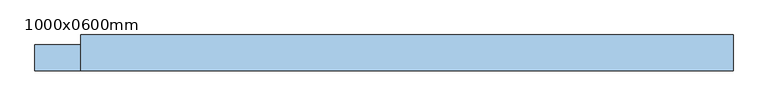
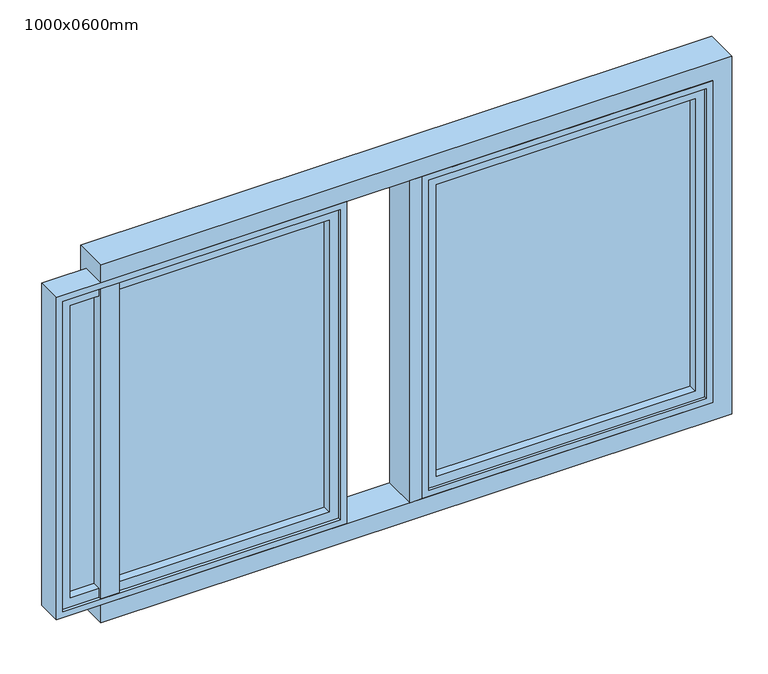
"""IFC4 building model written with IfcOpenShell, lengths in millimetres: window geometry, Janela Maxim-air - 2 Módulos : 1000x0600mm."""

from ifc_helpers import new_model, si_unit, frame, origin, place, context, project, spatial, polyline, outline, extrude, faceted_brep, source, transform, mapped, element, save


def window_1000x0600mm_9fc04acc(model_context):
    return source(origin(), model_context, "Body", "SolidModel", [
        extrude(outline(polyline([(452.0, 51.3), (28.0, 51.3), (28.0, 58.3), (452.0, 58.3), (452.0, 51.3)])), frame((0.0, 0.0, 1048.0), z_axis=(0.0, 0.0, 1.0), x_axis=(1.0, 0.0, 0.0)), (0.0, 0.0, 1.0), 504.0),
        faceted_brep([(35.0, 72.3, 1545.0), (35.0, 58.3, 1545.0), (35.0, 58.3, 1055.0), (35.0, 72.3, 1055.0), (28.0, 58.3, 1552.0), (28.0, 51.3, 1552.0), (28.0, 51.3, 1048.0), (28.0, 58.3, 1048.0), (35.0, 51.3, 1545.0), (35.0, 37.3, 1545.0), (35.0, 37.3, 1055.0), (35.0, 51.3, 1055.0), (15.0, 37.3, 1565.0), (15.0, 72.3, 1565.0), (15.0, 72.3, 1035.0), (15.0, 37.3, 1035.0), (445.0, 58.3, 1055.0), (445.0, 72.3, 1055.0), (452.0, 51.3, 1048.0), (452.0, 58.3, 1048.0), (445.0, 37.3, 1055.0), (445.0, 51.3, 1055.0), (465.0, 72.3, 1035.0), (465.0, 37.3, 1035.0), (445.0, 58.3, 1545.0), (445.0, 72.3, 1545.0), (452.0, 51.3, 1552.0), (452.0, 58.3, 1552.0), (445.0, 37.3, 1545.0), (445.0, 51.3, 1545.0), (465.0, 72.3, 1565.0), (465.0, 37.3, 1565.0)], [[[0, 1, 2, 3]], [[4, 5, 6, 7]], [[8, 9, 10, 11]], [[12, 13, 14, 15]], [[3, 2, 16, 17]], [[7, 6, 18, 19]], [[11, 10, 20, 21]], [[15, 14, 22, 23]], [[17, 16, 24, 25]], [[19, 18, 26, 27]], [[21, 20, 28, 29]], [[23, 22, 30, 31]], [[13, 30, 22, 14], [3, 17, 25, 0]], [[25, 24, 1, 0]], [[7, 19, 27, 4], [1, 24, 16, 2]], [[27, 26, 5, 4]], [[5, 26, 18, 6], [11, 21, 29, 8]], [[29, 28, 9, 8]], [[15, 23, 31, 12], [9, 28, 20, 10]], [[31, 30, 13, 12]]]),
        faceted_brep([(15.0, 72.3, 1565.0), (15.0, 37.3, 1565.0), (15.0, 37.3, 1035.0), (15.0, 72.3, 1035.0), (20.0, 37.3, 1560.0), (20.0, 32.3, 1560.0), (20.0, 32.3, 1040.0), (20.0, 37.3, 1040.0), (10.0, 32.3, 1570.0), (10.0, 72.3, 1570.0), (10.0, 72.3, 1030.0), (10.0, 32.3, 1030.0), (465.0, 37.3, 1035.0), (465.0, 72.3, 1035.0), (460.0, 32.3, 1040.0), (460.0, 37.3, 1040.0), (470.0, 72.3, 1030.0), (470.0, 32.3, 1030.0), (465.0, 37.3, 1565.0), (465.0, 72.3, 1565.0), (460.0, 32.3, 1560.0), (460.0, 37.3, 1560.0), (470.0, 72.3, 1570.0), (470.0, 32.3, 1570.0)], [[[0, 1, 2, 3]], [[4, 5, 6, 7]], [[8, 9, 10, 11]], [[3, 2, 12, 13]], [[7, 6, 14, 15]], [[11, 10, 16, 17]], [[13, 12, 18, 19]], [[15, 14, 20, 21]], [[17, 16, 22, 23]], [[9, 22, 16, 10], [3, 13, 19, 0]], [[19, 18, 1, 0]], [[1, 18, 12, 2], [7, 15, 21, 4]], [[21, 20, 5, 4]], [[11, 17, 23, 8], [5, 20, 14, 6]], [[23, 22, 9, 8]]]),
        extrude(outline(polyline([(-552.0, 51.3), (-552.0, 58.3), (-128.0, 58.3), (-128.0, 51.3), (-552.0, 51.3)])), frame((0.0, 0.0, 1048.0), z_axis=(0.0, 0.0, 1.0), x_axis=(1.0, 0.0, 0.0)), (0.0, 0.0, 1.0), 504.0),
        faceted_brep([(-135.0, 72.3, 1545.0), (-135.0, 72.3, 1055.0), (-135.0, 58.3, 1055.0), (-135.0, 58.3, 1545.0), (-128.0, 58.3, 1552.0), (-128.0, 58.3, 1048.0), (-128.0, 51.3, 1048.0), (-128.0, 51.3, 1552.0), (-135.0, 51.3, 1545.0), (-135.0, 51.3, 1055.0), (-135.0, 37.3, 1055.0), (-135.0, 37.3, 1545.0), (-115.0, 37.3, 1565.0), (-115.0, 37.3, 1035.0), (-115.0, 72.3, 1035.0), (-115.0, 72.3, 1565.0), (-545.0, 72.3, 1055.0), (-545.0, 58.3, 1055.0), (-552.0, 58.3, 1048.0), (-552.0, 51.3, 1048.0), (-545.0, 51.3, 1055.0), (-545.0, 37.3, 1055.0), (-565.0, 37.3, 1035.0), (-565.0, 72.3, 1035.0), (-545.0, 72.3, 1545.0), (-545.0, 58.3, 1545.0), (-552.0, 58.3, 1552.0), (-552.0, 51.3, 1552.0), (-545.0, 51.3, 1545.0), (-545.0, 37.3, 1545.0), (-565.0, 37.3, 1565.0), (-565.0, 72.3, 1565.0)], [[[0, 1, 2, 3]], [[4, 5, 6, 7]], [[8, 9, 10, 11]], [[12, 13, 14, 15]], [[1, 16, 17, 2]], [[5, 18, 19, 6]], [[9, 20, 21, 10]], [[13, 22, 23, 14]], [[16, 24, 25, 17]], [[18, 26, 27, 19]], [[20, 28, 29, 21]], [[22, 30, 31, 23]], [[15, 14, 23, 31], [1, 0, 24, 16]], [[24, 0, 3, 25]], [[5, 4, 26, 18], [3, 2, 17, 25]], [[26, 4, 7, 27]], [[7, 6, 19, 27], [9, 8, 28, 20]], [[28, 8, 11, 29]], [[13, 12, 30, 22], [11, 10, 21, 29]], [[30, 12, 15, 31]]]),
        faceted_brep([(-115.0, 72.3, 1565.0), (-115.0, 72.3, 1035.0), (-115.0, 37.3, 1035.0), (-115.0, 37.3, 1565.0), (-120.0, 37.3, 1560.0), (-120.0, 37.3, 1040.0), (-120.0, 32.3, 1040.0), (-120.0, 32.3, 1560.0), (-110.0, 32.3, 1570.0), (-110.0, 32.3, 1030.0), (-110.0, 72.3, 1030.0), (-110.0, 72.3, 1570.0), (-565.0, 72.3, 1035.0), (-565.0, 37.3, 1035.0), (-560.0, 37.3, 1040.0), (-560.0, 32.3, 1040.0), (-570.0, 32.3, 1030.0), (-570.0, 72.3, 1030.0), (-565.0, 72.3, 1565.0), (-565.0, 37.3, 1565.0), (-560.0, 37.3, 1560.0), (-560.0, 32.3, 1560.0), (-570.0, 32.3, 1570.0), (-570.0, 72.3, 1570.0)], [[[0, 1, 2, 3]], [[4, 5, 6, 7]], [[8, 9, 10, 11]], [[1, 12, 13, 2]], [[5, 14, 15, 6]], [[9, 16, 17, 10]], [[12, 18, 19, 13]], [[14, 20, 21, 15]], [[16, 22, 23, 17]], [[11, 10, 17, 23], [1, 0, 18, 12]], [[18, 0, 3, 19]], [[3, 2, 13, 19], [5, 4, 20, 14]], [[20, 4, 7, 21]], [[9, 8, 22, 16], [7, 6, 15, 21]], [[22, 8, 11, 23]]]),
        extrude(outline(polyline([(10.0, 87.3), (10.0, 32.3), (-10.0, 32.3), (-10.0, 87.3), (10.0, 87.3)])), frame((0.0, 0.0, 1030.0), z_axis=(0.0, 0.0, 1.0), x_axis=(1.0, 0.0, 0.0)), (0.0, 0.0, 1.0), 540.0),
        extrude(outline(polyline([(1000.0, 500.0), (1600.0, 500.0), (1600.0, -500.0), (1000.0, -500.0), (1000.0, 500.0)]), holes=[polyline([(1570.0, 470.0), (1030.0, 470.0), (1030.0, -470.0), (1570.0, -470.0), (1570.0, 470.0)])]), frame((0.0, 32.3, 0.0), z_axis=(0.0, 1.0, 0.0), x_axis=(0.0, 0.0, 1.0)), (0.0, 0.0, 1.0), 55.0),
    ])


if __name__ == "__main__":
    model = new_model("IFC4")
    model_context = context("Model", 3, world=origin())
    ifc_project = project(units=[si_unit("LENGTHUNIT", "METRE", prefix="MILLI")], contexts=[model_context])
    site = spatial("IfcSite", under=ifc_project)
    building = spatial("IfcBuilding", under=site)
    placement = place(None, origin())
    window_1000x0600mm_shape = window_1000x0600mm_9fc04acc(model_context)
    element("IfcWindow", 1, ObjectType="Janela Maxim-air - 2 Módulos : 1000x0600mm", at=placement, inside=building, context=model_context, shape_type="MappedRepresentation", body=[
        mapped(window_1000x0600mm_shape, transform((0.0, 0.0, 0.0), x_axis=(1.0, 0.0, 0.0), y_axis=(0.0, 1.0, 0.0), z_axis=(0.0, 0.0, 1.0))),
    ])
    save(model, "model.ifc")

# Revit data of these elements
# Type "Janela Maxim-air - 2 Módulos : 1000x0600mm"
#   Type Mark = "J12"
#   SINAPI = ""
#   ref. vert. basc. = 0.54 m
#   ref. horiz. basc. = 0.46 m
#   Largura Batente = 0.055 m
#   Height = 0.60 m
#   Default Sill Height = 1.00 m
#   Width = 1.00 m
#   Material Quadro = Metal - Alumínio
#   Material Painel = Vidro
#   Wall Closure = (empty or 0)
#   Assembly Code = ""
# Element 1 (IfcWindow, "Janela Maxim-air - 2 Módulos : 1000x0600mm")
#   Materials on its faces: "Metal - Alumínio", "Vidro"
# Materials
#   "Metal - Alumínio": class "Metal", colour RGB 244 244 244, transparency 0
#   "Vidro": class "Vidro", colour RGB 0 128 192, transparency 0.9, Description = "Vidro de sílica", Cost = 0
